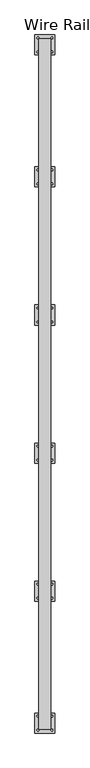
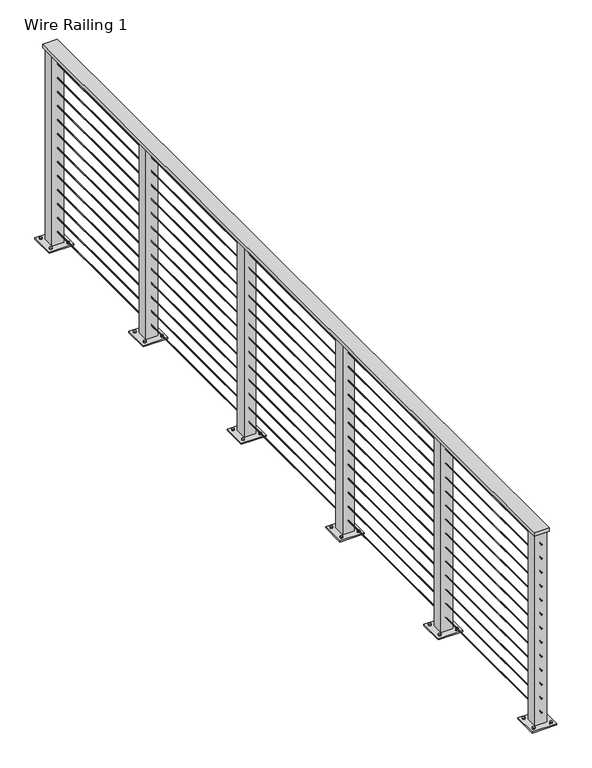
"""IFC4 building model written with IfcOpenShell, lengths in millimetres: railing geometry, Wire Railing 1."""

from ifc_helpers import new_model, si_unit, point, frame, frame_2d, origin, place, context, project, spatial, polyline, circle_curve, trimmed, segment, composite_curve, outline, extrude, source, transform, mapped, element, save


def wire_railing_1_9cbc15e5(model_context):
    return source(origin(), model_context, "Body", "SweptSolid", [
        extrude(outline(polyline([(33186.6840778, 35259.9668167), (33262.8840778, 35259.9668167), (33262.8840778, 30878.4668167), (33186.6840778, 30878.4668167), (33186.6840778, 35259.9668167)])), frame((0.0, 0.0, 270306.8), z_axis=(0.0, 0.0, 1.0), x_axis=(1.0, 0.0, 0.0)), (0.0, 0.0, 1.0), 19.05),
        extrude(outline(composite_curve([segment(trimmed(circle_curve(frame_2d((270247.26875, 33224.7840778)), 2.38125), [point((270247.26875, 33227.1653278))], [point((270247.26875, 33222.4028278))], False, "CARTESIAN"), True, "CONTINUOUS"), segment(trimmed(circle_curve(frame_2d((270247.26875, 33224.7840778)), 2.38125), [point((270247.26875, 33222.4028278))], [point((270247.26875, 33227.1653278))], False, "CARTESIAN"), True, "CONTINUOUS")], self_intersect=False)), frame((0.0, 30878.4668167, 0.0), z_axis=(0.0, 1.0, 0.0), x_axis=(0.0, 0.0, 1.0)), (0.0, 0.0, 1.0), 4381.5),
        extrude(outline(composite_curve([segment(trimmed(circle_curve(frame_2d((270171.06875, 33224.7840778)), 2.38125), [point((270171.06875, 33227.1653278))], [point((270171.06875, 33222.4028278))], False, "CARTESIAN"), True, "CONTINUOUS"), segment(trimmed(circle_curve(frame_2d((270171.06875, 33224.7840778)), 2.38125), [point((270171.06875, 33222.4028278))], [point((270171.06875, 33227.1653278))], False, "CARTESIAN"), True, "CONTINUOUS")], self_intersect=False)), frame((0.0, 30878.4668167, 0.0), z_axis=(0.0, 1.0, 0.0), x_axis=(0.0, 0.0, 1.0)), (0.0, 0.0, 1.0), 4381.5),
        extrude(outline(composite_curve([segment(trimmed(circle_curve(frame_2d((270094.86875, 33224.7840778)), 2.38125), [point((270094.86875, 33227.1653278))], [point((270094.86875, 33222.4028278))], False, "CARTESIAN"), True, "CONTINUOUS"), segment(trimmed(circle_curve(frame_2d((270094.86875, 33224.7840778)), 2.38125), [point((270094.86875, 33222.4028278))], [point((270094.86875, 33227.1653278))], False, "CARTESIAN"), True, "CONTINUOUS")], self_intersect=False)), frame((0.0, 30878.4668167, 0.0), z_axis=(0.0, 1.0, 0.0), x_axis=(0.0, 0.0, 1.0)), (0.0, 0.0, 1.0), 4381.5),
        extrude(outline(composite_curve([segment(trimmed(circle_curve(frame_2d((270018.66875, 33224.7840778)), 2.38125), [point((270018.66875, 33227.1653278))], [point((270018.66875, 33222.4028278))], False, "CARTESIAN"), True, "CONTINUOUS"), segment(trimmed(circle_curve(frame_2d((270018.66875, 33224.7840778)), 2.38125), [point((270018.66875, 33222.4028278))], [point((270018.66875, 33227.1653278))], False, "CARTESIAN"), True, "CONTINUOUS")], self_intersect=False)), frame((0.0, 30878.4668167, 0.0), z_axis=(0.0, 1.0, 0.0), x_axis=(0.0, 0.0, 1.0)), (0.0, 0.0, 1.0), 4381.5),
        extrude(outline(composite_curve([segment(trimmed(circle_curve(frame_2d((269942.46875, 33224.7840778)), 2.38125), [point((269942.46875, 33227.1653278))], [point((269942.46875, 33222.4028278))], False, "CARTESIAN"), True, "CONTINUOUS"), segment(trimmed(circle_curve(frame_2d((269942.46875, 33224.7840778)), 2.38125), [point((269942.46875, 33222.4028278))], [point((269942.46875, 33227.1653278))], False, "CARTESIAN"), True, "CONTINUOUS")], self_intersect=False)), frame((0.0, 30878.4668167, 0.0), z_axis=(0.0, 1.0, 0.0), x_axis=(0.0, 0.0, 1.0)), (0.0, 0.0, 1.0), 4381.5),
        extrude(outline(composite_curve([segment(trimmed(circle_curve(frame_2d((269866.26875, 33224.7840778)), 2.38125), [point((269866.26875, 33227.1653278))], [point((269866.26875, 33222.4028278))], False, "CARTESIAN"), True, "CONTINUOUS"), segment(trimmed(circle_curve(frame_2d((269866.26875, 33224.7840778)), 2.38125), [point((269866.26875, 33222.4028278))], [point((269866.26875, 33227.1653278))], False, "CARTESIAN"), True, "CONTINUOUS")], self_intersect=False)), frame((0.0, 30878.4668167, 0.0), z_axis=(0.0, 1.0, 0.0), x_axis=(0.0, 0.0, 1.0)), (0.0, 0.0, 1.0), 4381.5),
        extrude(outline(composite_curve([segment(trimmed(circle_curve(frame_2d((269790.06875, 33224.7840778)), 2.38125), [point((269790.06875, 33227.1653278))], [point((269790.06875, 33222.4028278))], False, "CARTESIAN"), True, "CONTINUOUS"), segment(trimmed(circle_curve(frame_2d((269790.06875, 33224.7840778)), 2.38125), [point((269790.06875, 33222.4028278))], [point((269790.06875, 33227.1653278))], False, "CARTESIAN"), True, "CONTINUOUS")], self_intersect=False)), frame((0.0, 30878.4668167, 0.0), z_axis=(0.0, 1.0, 0.0), x_axis=(0.0, 0.0, 1.0)), (0.0, 0.0, 1.0), 4381.5),
        extrude(outline(composite_curve([segment(trimmed(circle_curve(frame_2d((269713.86875, 33224.7840778)), 2.38125), [point((269713.86875, 33227.1653278))], [point((269713.86875, 33222.4028278))], False, "CARTESIAN"), True, "CONTINUOUS"), segment(trimmed(circle_curve(frame_2d((269713.86875, 33224.7840778)), 2.38125), [point((269713.86875, 33222.4028278))], [point((269713.86875, 33227.1653278))], False, "CARTESIAN"), True, "CONTINUOUS")], self_intersect=False)), frame((0.0, 30878.4668167, 0.0), z_axis=(0.0, 1.0, 0.0), x_axis=(0.0, 0.0, 1.0)), (0.0, 0.0, 1.0), 4381.5),
        extrude(outline(composite_curve([segment(trimmed(circle_curve(frame_2d((269637.66875, 33224.7840778)), 2.38125), [point((269637.66875, 33227.1653278))], [point((269637.66875, 33222.4028278))], False, "CARTESIAN"), True, "CONTINUOUS"), segment(trimmed(circle_curve(frame_2d((269637.66875, 33224.7840778)), 2.38125), [point((269637.66875, 33222.4028278))], [point((269637.66875, 33227.1653278))], False, "CARTESIAN"), True, "CONTINUOUS")], self_intersect=False)), frame((0.0, 30878.4668167, 0.0), z_axis=(0.0, 1.0, 0.0), x_axis=(0.0, 0.0, 1.0)), (0.0, 0.0, 1.0), 4381.5),
        extrude(outline(composite_curve([segment(trimmed(circle_curve(frame_2d((269561.46875, 33224.7840778)), 2.38125), [point((269561.46875, 33227.1653278))], [point((269561.46875, 33222.4028278))], False, "CARTESIAN"), True, "CONTINUOUS"), segment(trimmed(circle_curve(frame_2d((269561.46875, 33224.7840778)), 2.38125), [point((269561.46875, 33222.4028278))], [point((269561.46875, 33227.1653278))], False, "CARTESIAN"), True, "CONTINUOUS")], self_intersect=False)), frame((0.0, 30878.4668167, 0.0), z_axis=(0.0, 1.0, 0.0), x_axis=(0.0, 0.0, 1.0)), (0.0, 0.0, 1.0), 4381.5),
        extrude(outline(composite_curve([segment(trimmed(circle_curve(frame_2d((269485.26875, 33224.7840778)), 2.38125), [point((269485.26875, 33227.1653278))], [point((269485.26875, 33222.4028278))], False, "CARTESIAN"), True, "CONTINUOUS"), segment(trimmed(circle_curve(frame_2d((269485.26875, 33224.7840778)), 2.38125), [point((269485.26875, 33222.4028278))], [point((269485.26875, 33227.1653278))], False, "CARTESIAN"), True, "CONTINUOUS")], self_intersect=False)), frame((0.0, 30878.4668167, 0.0), z_axis=(0.0, 1.0, 0.0), x_axis=(0.0, 0.0, 1.0)), (0.0, 0.0, 1.0), 4381.5),
        extrude(outline(composite_curve([segment(trimmed(circle_curve(frame_2d((269409.06875, 33224.7840778)), 2.38125), [point((269409.06875, 33227.1653278))], [point((269409.06875, 33222.4028278))], False, "CARTESIAN"), True, "CONTINUOUS"), segment(trimmed(circle_curve(frame_2d((269409.06875, 33224.7840778)), 2.38125), [point((269409.06875, 33222.4028278))], [point((269409.06875, 33227.1653278))], False, "CARTESIAN"), True, "CONTINUOUS")], self_intersect=False)), frame((0.0, 30878.4668167, 0.0), z_axis=(0.0, 1.0, 0.0), x_axis=(0.0, 0.0, 1.0)), (0.0, 0.0, 1.0), 4381.5),
        extrude(outline(composite_curve([segment(trimmed(circle_curve(frame_2d((269332.86875, 33224.7840778)), 2.38125), [point((269332.86875, 33227.1653278))], [point((269332.86875, 33222.4028278))], False, "CARTESIAN"), True, "CONTINUOUS"), segment(trimmed(circle_curve(frame_2d((269332.86875, 33224.7840778)), 2.38125), [point((269332.86875, 33222.4028278))], [point((269332.86875, 33227.1653278))], False, "CARTESIAN"), True, "CONTINUOUS")], self_intersect=False)), frame((0.0, 30878.4668167, 0.0), z_axis=(0.0, 1.0, 0.0), x_axis=(0.0, 0.0, 1.0)), (0.0, 0.0, 1.0), 4381.5),
        extrude(outline(composite_curve([segment(trimmed(circle_curve(frame_2d((33180.3340778, 31799.2168167)), 6.35), [point((33173.9840778, 31799.2168167))], [point((33186.6840778, 31799.2168167))], False, "CARTESIAN"), True, "CONTINUOUS"), segment(trimmed(circle_curve(frame_2d((33180.3340778, 31799.2168167)), 6.35), [point((33186.6840778, 31799.2168167))], [point((33173.9840778, 31799.2168167))], False, "CARTESIAN"), True, "CONTINUOUS")], self_intersect=False)), frame((0.0, 0.0, 269259.05), z_axis=(0.0, 0.0, 1.0), x_axis=(1.0, 0.0, 0.0)), (0.0, 0.0, 1.0), 12.7),
        extrude(outline(composite_curve([segment(trimmed(circle_curve(frame_2d((33269.2340778, 31799.2168167)), 6.35), [point((33262.8840778, 31799.2168167))], [point((33275.5840778, 31799.2168167))], False, "CARTESIAN"), True, "CONTINUOUS"), segment(trimmed(circle_curve(frame_2d((33269.2340778, 31799.2168167)), 6.35), [point((33275.5840778, 31799.2168167))], [point((33262.8840778, 31799.2168167))], False, "CARTESIAN"), True, "CONTINUOUS")], self_intersect=False)), frame((0.0, 0.0, 269259.05), z_axis=(0.0, 0.0, 1.0), x_axis=(1.0, 0.0, 0.0)), (0.0, 0.0, 1.0), 12.7),
        extrude(outline(composite_curve([segment(trimmed(circle_curve(frame_2d((33180.3340778, 31710.3168167)), 6.35), [point((33173.9840778, 31710.3168167))], [point((33186.6840778, 31710.3168167))], False, "CARTESIAN"), True, "CONTINUOUS"), segment(trimmed(circle_curve(frame_2d((33180.3340778, 31710.3168167)), 6.35), [point((33186.6840778, 31710.3168167))], [point((33173.9840778, 31710.3168167))], False, "CARTESIAN"), True, "CONTINUOUS")], self_intersect=False)), frame((0.0, 0.0, 269259.05), z_axis=(0.0, 0.0, 1.0), x_axis=(1.0, 0.0, 0.0)), (0.0, 0.0, 1.0), 12.7),
        extrude(outline(composite_curve([segment(trimmed(circle_curve(frame_2d((33269.2340778, 31710.3168167)), 6.35), [point((33262.8840778, 31710.3168167))], [point((33275.5840778, 31710.3168167))], False, "CARTESIAN"), True, "CONTINUOUS"), segment(trimmed(circle_curve(frame_2d((33269.2340778, 31710.3168167)), 6.35), [point((33275.5840778, 31710.3168167))], [point((33262.8840778, 31710.3168167))], False, "CARTESIAN"), True, "CONTINUOUS")], self_intersect=False)), frame((0.0, 0.0, 269259.05), z_axis=(0.0, 0.0, 1.0), x_axis=(1.0, 0.0, 0.0)), (0.0, 0.0, 1.0), 12.7),
        extrude(outline(polyline([(33288.2840778, 31818.2668167), (33288.2840778, 31691.2668167), (33161.2840778, 31691.2668167), (33161.2840778, 31818.2668167), (33288.2840778, 31818.2668167)])), frame((0.0, 0.0, 269259.05), z_axis=(0.0, 0.0, 1.0), x_axis=(1.0, 0.0, 0.0)), (0.0, 0.0, 1.0), 6.35),
        extrude(outline(polyline([(33254.9465778, 31784.9293167), (33254.9465778, 31724.6043167), (33194.6215778, 31724.6043167), (33194.6215778, 31784.9293167), (33254.9465778, 31784.9293167)]), holes=[polyline([(33248.5965778, 31778.5793167), (33200.9715778, 31778.5793167), (33200.9715778, 31730.9543167), (33248.5965778, 31730.9543167), (33248.5965778, 31778.5793167)])]), frame((0.0, 0.0, 269259.05), z_axis=(0.0, 0.0, 1.0), x_axis=(1.0, 0.0, 0.0)), (0.0, 0.0, 1.0), 1047.75),
        extrude(outline(composite_curve([segment(trimmed(circle_curve(frame_2d((33180.3340778, 32675.5168167)), 6.35), [point((33173.9840778, 32675.5168167))], [point((33186.6840778, 32675.5168167))], False, "CARTESIAN"), True, "CONTINUOUS"), segment(trimmed(circle_curve(frame_2d((33180.3340778, 32675.5168167)), 6.35), [point((33186.6840778, 32675.5168167))], [point((33173.9840778, 32675.5168167))], False, "CARTESIAN"), True, "CONTINUOUS")], self_intersect=False)), frame((0.0, 0.0, 269259.05), z_axis=(0.0, 0.0, 1.0), x_axis=(1.0, 0.0, 0.0)), (0.0, 0.0, 1.0), 12.7),
        extrude(outline(composite_curve([segment(trimmed(circle_curve(frame_2d((33269.2340778, 32675.5168167)), 6.35), [point((33262.8840778, 32675.5168167))], [point((33275.5840778, 32675.5168167))], False, "CARTESIAN"), True, "CONTINUOUS"), segment(trimmed(circle_curve(frame_2d((33269.2340778, 32675.5168167)), 6.35), [point((33275.5840778, 32675.5168167))], [point((33262.8840778, 32675.5168167))], False, "CARTESIAN"), True, "CONTINUOUS")], self_intersect=False)), frame((0.0, 0.0, 269259.05), z_axis=(0.0, 0.0, 1.0), x_axis=(1.0, 0.0, 0.0)), (0.0, 0.0, 1.0), 12.7),
        extrude(outline(composite_curve([segment(trimmed(circle_curve(frame_2d((33180.3340778, 32586.6168167)), 6.35), [point((33173.9840778, 32586.6168167))], [point((33186.6840778, 32586.6168167))], False, "CARTESIAN"), True, "CONTINUOUS"), segment(trimmed(circle_curve(frame_2d((33180.3340778, 32586.6168167)), 6.35), [point((33186.6840778, 32586.6168167))], [point((33173.9840778, 32586.6168167))], False, "CARTESIAN"), True, "CONTINUOUS")], self_intersect=False)), frame((0.0, 0.0, 269259.05), z_axis=(0.0, 0.0, 1.0), x_axis=(1.0, 0.0, 0.0)), (0.0, 0.0, 1.0), 12.7),
        extrude(outline(composite_curve([segment(trimmed(circle_curve(frame_2d((33269.2340778, 32586.6168167)), 6.35), [point((33262.8840778, 32586.6168167))], [point((33275.5840778, 32586.6168167))], False, "CARTESIAN"), True, "CONTINUOUS"), segment(trimmed(circle_curve(frame_2d((33269.2340778, 32586.6168167)), 6.35), [point((33275.5840778, 32586.6168167))], [point((33262.8840778, 32586.6168167))], False, "CARTESIAN"), True, "CONTINUOUS")], self_intersect=False)), frame((0.0, 0.0, 269259.05), z_axis=(0.0, 0.0, 1.0), x_axis=(1.0, 0.0, 0.0)), (0.0, 0.0, 1.0), 12.7),
        extrude(outline(polyline([(33288.2840778, 32694.5668167), (33288.2840778, 32567.5668167), (33161.2840778, 32567.5668167), (33161.2840778, 32694.5668167), (33288.2840778, 32694.5668167)])), frame((0.0, 0.0, 269259.05), z_axis=(0.0, 0.0, 1.0), x_axis=(1.0, 0.0, 0.0)), (0.0, 0.0, 1.0), 6.35),
        extrude(outline(polyline([(33254.9465778, 32661.2293167), (33254.9465778, 32600.9043167), (33194.6215778, 32600.9043167), (33194.6215778, 32661.2293167), (33254.9465778, 32661.2293167)]), holes=[polyline([(33248.5965778, 32654.8793167), (33200.9715778, 32654.8793167), (33200.9715778, 32607.2543167), (33248.5965778, 32607.2543167), (33248.5965778, 32654.8793167)])]), frame((0.0, 0.0, 269259.05), z_axis=(0.0, 0.0, 1.0), x_axis=(1.0, 0.0, 0.0)), (0.0, 0.0, 1.0), 1047.75),
        extrude(outline(composite_curve([segment(trimmed(circle_curve(frame_2d((33180.3340778, 33551.8168167)), 6.35), [point((33173.9840778, 33551.8168167))], [point((33186.6840778, 33551.8168167))], False, "CARTESIAN"), True, "CONTINUOUS"), segment(trimmed(circle_curve(frame_2d((33180.3340778, 33551.8168167)), 6.35), [point((33186.6840778, 33551.8168167))], [point((33173.9840778, 33551.8168167))], False, "CARTESIAN"), True, "CONTINUOUS")], self_intersect=False)), frame((0.0, 0.0, 269259.05), z_axis=(0.0, 0.0, 1.0), x_axis=(1.0, 0.0, 0.0)), (0.0, 0.0, 1.0), 12.7),
        extrude(outline(composite_curve([segment(trimmed(circle_curve(frame_2d((33269.2340778, 33551.8168167)), 6.35), [point((33262.8840778, 33551.8168167))], [point((33275.5840778, 33551.8168167))], False, "CARTESIAN"), True, "CONTINUOUS"), segment(trimmed(circle_curve(frame_2d((33269.2340778, 33551.8168167)), 6.35), [point((33275.5840778, 33551.8168167))], [point((33262.8840778, 33551.8168167))], False, "CARTESIAN"), True, "CONTINUOUS")], self_intersect=False)), frame((0.0, 0.0, 269259.05), z_axis=(0.0, 0.0, 1.0), x_axis=(1.0, 0.0, 0.0)), (0.0, 0.0, 1.0), 12.7),
        extrude(outline(composite_curve([segment(trimmed(circle_curve(frame_2d((33180.3340778, 33462.9168167)), 6.35), [point((33173.9840778, 33462.9168167))], [point((33186.6840778, 33462.9168167))], False, "CARTESIAN"), True, "CONTINUOUS"), segment(trimmed(circle_curve(frame_2d((33180.3340778, 33462.9168167)), 6.35), [point((33186.6840778, 33462.9168167))], [point((33173.9840778, 33462.9168167))], False, "CARTESIAN"), True, "CONTINUOUS")], self_intersect=False)), frame((0.0, 0.0, 269259.05), z_axis=(0.0, 0.0, 1.0), x_axis=(1.0, 0.0, 0.0)), (0.0, 0.0, 1.0), 12.7),
        extrude(outline(composite_curve([segment(trimmed(circle_curve(frame_2d((33269.2340778, 33462.9168167)), 6.35), [point((33262.8840778, 33462.9168167))], [point((33275.5840778, 33462.9168167))], False, "CARTESIAN"), True, "CONTINUOUS"), segment(trimmed(circle_curve(frame_2d((33269.2340778, 33462.9168167)), 6.35), [point((33275.5840778, 33462.9168167))], [point((33262.8840778, 33462.9168167))], False, "CARTESIAN"), True, "CONTINUOUS")], self_intersect=False)), frame((0.0, 0.0, 269259.05), z_axis=(0.0, 0.0, 1.0), x_axis=(1.0, 0.0, 0.0)), (0.0, 0.0, 1.0), 12.7),
        extrude(outline(polyline([(33288.2840778, 33570.8668167), (33288.2840778, 33443.8668167), (33161.2840778, 33443.8668167), (33161.2840778, 33570.8668167), (33288.2840778, 33570.8668167)])), frame((0.0, 0.0, 269259.05), z_axis=(0.0, 0.0, 1.0), x_axis=(1.0, 0.0, 0.0)), (0.0, 0.0, 1.0), 6.35),
        extrude(outline(polyline([(33254.9465778, 33537.5293167), (33254.9465778, 33477.2043167), (33194.6215778, 33477.2043167), (33194.6215778, 33537.5293167), (33254.9465778, 33537.5293167)]), holes=[polyline([(33248.5965778, 33531.1793167), (33200.9715778, 33531.1793167), (33200.9715778, 33483.5543167), (33248.5965778, 33483.5543167), (33248.5965778, 33531.1793167)])]), frame((0.0, 0.0, 269259.05), z_axis=(0.0, 0.0, 1.0), x_axis=(1.0, 0.0, 0.0)), (0.0, 0.0, 1.0), 1047.75),
        extrude(outline(composite_curve([segment(trimmed(circle_curve(frame_2d((33180.3340778, 34428.1168167)), 6.35), [point((33173.9840778, 34428.1168167))], [point((33186.6840778, 34428.1168167))], False, "CARTESIAN"), True, "CONTINUOUS"), segment(trimmed(circle_curve(frame_2d((33180.3340778, 34428.1168167)), 6.35), [point((33186.6840778, 34428.1168167))], [point((33173.9840778, 34428.1168167))], False, "CARTESIAN"), True, "CONTINUOUS")], self_intersect=False)), frame((0.0, 0.0, 269259.05), z_axis=(0.0, 0.0, 1.0), x_axis=(1.0, 0.0, 0.0)), (0.0, 0.0, 1.0), 12.7),
        extrude(outline(composite_curve([segment(trimmed(circle_curve(frame_2d((33269.2340778, 34428.1168167)), 6.35), [point((33262.8840778, 34428.1168167))], [point((33275.5840778, 34428.1168167))], False, "CARTESIAN"), True, "CONTINUOUS"), segment(trimmed(circle_curve(frame_2d((33269.2340778, 34428.1168167)), 6.35), [point((33275.5840778, 34428.1168167))], [point((33262.8840778, 34428.1168167))], False, "CARTESIAN"), True, "CONTINUOUS")], self_intersect=False)), frame((0.0, 0.0, 269259.05), z_axis=(0.0, 0.0, 1.0), x_axis=(1.0, 0.0, 0.0)), (0.0, 0.0, 1.0), 12.7),
        extrude(outline(composite_curve([segment(trimmed(circle_curve(frame_2d((33180.3340778, 34339.2168167)), 6.35), [point((33173.9840778, 34339.2168167))], [point((33186.6840778, 34339.2168167))], False, "CARTESIAN"), True, "CONTINUOUS"), segment(trimmed(circle_curve(frame_2d((33180.3340778, 34339.2168167)), 6.35), [point((33186.6840778, 34339.2168167))], [point((33173.9840778, 34339.2168167))], False, "CARTESIAN"), True, "CONTINUOUS")], self_intersect=False)), frame((0.0, 0.0, 269259.05), z_axis=(0.0, 0.0, 1.0), x_axis=(1.0, 0.0, 0.0)), (0.0, 0.0, 1.0), 12.7),
        extrude(outline(composite_curve([segment(trimmed(circle_curve(frame_2d((33269.2340778, 34339.2168167)), 6.35), [point((33262.8840778, 34339.2168167))], [point((33275.5840778, 34339.2168167))], False, "CARTESIAN"), True, "CONTINUOUS"), segment(trimmed(circle_curve(frame_2d((33269.2340778, 34339.2168167)), 6.35), [point((33275.5840778, 34339.2168167))], [point((33262.8840778, 34339.2168167))], False, "CARTESIAN"), True, "CONTINUOUS")], self_intersect=False)), frame((0.0, 0.0, 269259.05), z_axis=(0.0, 0.0, 1.0), x_axis=(1.0, 0.0, 0.0)), (0.0, 0.0, 1.0), 12.7),
        extrude(outline(polyline([(33288.2840778, 34447.1668167), (33288.2840778, 34320.1668167), (33161.2840778, 34320.1668167), (33161.2840778, 34447.1668167), (33288.2840778, 34447.1668167)])), frame((0.0, 0.0, 269259.05), z_axis=(0.0, 0.0, 1.0), x_axis=(1.0, 0.0, 0.0)), (0.0, 0.0, 1.0), 6.35),
        extrude(outline(polyline([(33254.9465778, 34413.8293167), (33254.9465778, 34353.5043167), (33194.6215778, 34353.5043167), (33194.6215778, 34413.8293167), (33254.9465778, 34413.8293167)]), holes=[polyline([(33248.5965778, 34407.4793167), (33200.9715778, 34407.4793167), (33200.9715778, 34359.8543167), (33248.5965778, 34359.8543167), (33248.5965778, 34407.4793167)])]), frame((0.0, 0.0, 269259.05), z_axis=(0.0, 0.0, 1.0), x_axis=(1.0, 0.0, 0.0)), (0.0, 0.0, 1.0), 1047.75),
        extrude(outline(composite_curve([segment(trimmed(circle_curve(frame_2d((33180.3340778, 30961.0168167)), 6.35), [point((33173.9840778, 30961.0168167))], [point((33186.6840778, 30961.0168167))], False, "CARTESIAN"), True, "CONTINUOUS"), segment(trimmed(circle_curve(frame_2d((33180.3340778, 30961.0168167)), 6.35), [point((33186.6840778, 30961.0168167))], [point((33173.9840778, 30961.0168167))], False, "CARTESIAN"), True, "CONTINUOUS")], self_intersect=False)), frame((0.0, 0.0, 269259.05), z_axis=(0.0, 0.0, 1.0), x_axis=(1.0, 0.0, 0.0)), (0.0, 0.0, 1.0), 12.7),
        extrude(outline(composite_curve([segment(trimmed(circle_curve(frame_2d((33269.2340778, 30961.0168167)), 6.35), [point((33262.8840778, 30961.0168167))], [point((33275.5840778, 30961.0168167))], False, "CARTESIAN"), True, "CONTINUOUS"), segment(trimmed(circle_curve(frame_2d((33269.2340778, 30961.0168167)), 6.35), [point((33275.5840778, 30961.0168167))], [point((33262.8840778, 30961.0168167))], False, "CARTESIAN"), True, "CONTINUOUS")], self_intersect=False)), frame((0.0, 0.0, 269259.05), z_axis=(0.0, 0.0, 1.0), x_axis=(1.0, 0.0, 0.0)), (0.0, 0.0, 1.0), 12.7),
        extrude(outline(composite_curve([segment(trimmed(circle_curve(frame_2d((33180.3340778, 30872.1168167)), 6.35), [point((33173.9840778, 30872.1168167))], [point((33186.6840778, 30872.1168167))], False, "CARTESIAN"), True, "CONTINUOUS"), segment(trimmed(circle_curve(frame_2d((33180.3340778, 30872.1168167)), 6.35), [point((33186.6840778, 30872.1168167))], [point((33173.9840778, 30872.1168167))], False, "CARTESIAN"), True, "CONTINUOUS")], self_intersect=False)), frame((0.0, 0.0, 269259.05), z_axis=(0.0, 0.0, 1.0), x_axis=(1.0, 0.0, 0.0)), (0.0, 0.0, 1.0), 12.7),
        extrude(outline(composite_curve([segment(trimmed(circle_curve(frame_2d((33269.2340778, 30872.1168167)), 6.35), [point((33262.8840778, 30872.1168167))], [point((33275.5840778, 30872.1168167))], False, "CARTESIAN"), True, "CONTINUOUS"), segment(trimmed(circle_curve(frame_2d((33269.2340778, 30872.1168167)), 6.35), [point((33275.5840778, 30872.1168167))], [point((33262.8840778, 30872.1168167))], False, "CARTESIAN"), True, "CONTINUOUS")], self_intersect=False)), frame((0.0, 0.0, 269259.05), z_axis=(0.0, 0.0, 1.0), x_axis=(1.0, 0.0, 0.0)), (0.0, 0.0, 1.0), 12.7),
        extrude(outline(polyline([(33288.2840778, 30980.0668167), (33288.2840778, 30853.0668167), (33161.2840778, 30853.0668167), (33161.2840778, 30980.0668167), (33288.2840778, 30980.0668167)])), frame((0.0, 0.0, 269259.05), z_axis=(0.0, 0.0, 1.0), x_axis=(1.0, 0.0, 0.0)), (0.0, 0.0, 1.0), 6.35),
        extrude(outline(polyline([(33254.9465778, 30946.7293167), (33254.9465778, 30886.4043167), (33194.6215778, 30886.4043167), (33194.6215778, 30946.7293167), (33254.9465778, 30946.7293167)]), holes=[polyline([(33248.5965778, 30940.3793167), (33200.9715778, 30940.3793167), (33200.9715778, 30892.7543167), (33248.5965778, 30892.7543167), (33248.5965778, 30940.3793167)])]), frame((0.0, 0.0, 269259.05), z_axis=(0.0, 0.0, 1.0), x_axis=(1.0, 0.0, 0.0)), (0.0, 0.0, 1.0), 1047.75),
        extrude(outline(composite_curve([segment(trimmed(circle_curve(frame_2d((33180.3340778, 35266.3168167)), 6.35), [point((33173.9840778, 35266.3168167))], [point((33186.6840778, 35266.3168167))], False, "CARTESIAN"), True, "CONTINUOUS"), segment(trimmed(circle_curve(frame_2d((33180.3340778, 35266.3168167)), 6.35), [point((33186.6840778, 35266.3168167))], [point((33173.9840778, 35266.3168167))], False, "CARTESIAN"), True, "CONTINUOUS")], self_intersect=False)), frame((0.0, 0.0, 269259.05), z_axis=(0.0, 0.0, 1.0), x_axis=(1.0, 0.0, 0.0)), (0.0, 0.0, 1.0), 12.7),
        extrude(outline(composite_curve([segment(trimmed(circle_curve(frame_2d((33269.2340778, 35266.3168167)), 6.35), [point((33262.8840778, 35266.3168167))], [point((33275.5840778, 35266.3168167))], False, "CARTESIAN"), True, "CONTINUOUS"), segment(trimmed(circle_curve(frame_2d((33269.2340778, 35266.3168167)), 6.35), [point((33275.5840778, 35266.3168167))], [point((33262.8840778, 35266.3168167))], False, "CARTESIAN"), True, "CONTINUOUS")], self_intersect=False)), frame((0.0, 0.0, 269259.05), z_axis=(0.0, 0.0, 1.0), x_axis=(1.0, 0.0, 0.0)), (0.0, 0.0, 1.0), 12.7),
        extrude(outline(composite_curve([segment(trimmed(circle_curve(frame_2d((33180.3340778, 35177.4168167)), 6.35), [point((33173.9840778, 35177.4168167))], [point((33186.6840778, 35177.4168167))], False, "CARTESIAN"), True, "CONTINUOUS"), segment(trimmed(circle_curve(frame_2d((33180.3340778, 35177.4168167)), 6.35), [point((33186.6840778, 35177.4168167))], [point((33173.9840778, 35177.4168167))], False, "CARTESIAN"), True, "CONTINUOUS")], self_intersect=False)), frame((0.0, 0.0, 269259.05), z_axis=(0.0, 0.0, 1.0), x_axis=(1.0, 0.0, 0.0)), (0.0, 0.0, 1.0), 12.7),
        extrude(outline(composite_curve([segment(trimmed(circle_curve(frame_2d((33269.2340778, 35177.4168167)), 6.35), [point((33262.8840778, 35177.4168167))], [point((33275.5840778, 35177.4168167))], False, "CARTESIAN"), True, "CONTINUOUS"), segment(trimmed(circle_curve(frame_2d((33269.2340778, 35177.4168167)), 6.35), [point((33275.5840778, 35177.4168167))], [point((33262.8840778, 35177.4168167))], False, "CARTESIAN"), True, "CONTINUOUS")], self_intersect=False)), frame((0.0, 0.0, 269259.05), z_axis=(0.0, 0.0, 1.0), x_axis=(1.0, 0.0, 0.0)), (0.0, 0.0, 1.0), 12.7),
        extrude(outline(polyline([(33288.2840778, 35285.3668167), (33288.2840778, 35158.3668167), (33161.2840778, 35158.3668167), (33161.2840778, 35285.3668167), (33288.2840778, 35285.3668167)])), frame((0.0, 0.0, 269259.05), z_axis=(0.0, 0.0, 1.0), x_axis=(1.0, 0.0, 0.0)), (0.0, 0.0, 1.0), 6.35),
        extrude(outline(polyline([(33254.9465778, 35252.0293167), (33254.9465778, 35191.7043167), (33194.6215778, 35191.7043167), (33194.6215778, 35252.0293167), (33254.9465778, 35252.0293167)]), holes=[polyline([(33248.5965778, 35245.6793167), (33200.9715778, 35245.6793167), (33200.9715778, 35198.0543167), (33248.5965778, 35198.0543167), (33248.5965778, 35245.6793167)])]), frame((0.0, 0.0, 269259.05), z_axis=(0.0, 0.0, 1.0), x_axis=(1.0, 0.0, 0.0)), (0.0, 0.0, 1.0), 1047.75),
    ])


if __name__ == "__main__":
    model = new_model("IFC4")
    model_context = context("Model", 3, world=origin())
    ifc_project = project(units=[si_unit("LENGTHUNIT", "METRE", prefix="MILLI")], contexts=[model_context])
    site = spatial("IfcSite", under=ifc_project)
    building = spatial("IfcBuilding", under=site)
    placement = place(None, origin())
    wire_railing_1_shape = wire_railing_1_9cbc15e5(model_context)
    element("IfcRailing", 1, ObjectType="Wire Railing 1", at=placement, inside=building, context=model_context, shape_type="MappedRepresentation", body=[
        mapped(wire_railing_1_shape, transform((0.0, 0.0, 0.0), x_axis=(1.0, 0.0, 0.0), y_axis=(0.0, 1.0, 0.0), z_axis=(0.0, 0.0, 1.0))),
    ])
    save(model, "model.ifc")

# Revit data of these elements
# Element 1 (IfcRailing, "Wire Railing 1")
#   Materials on its faces: "2 1/2\" X 2 1/2\" ALUM. SQUARE POST (38\" O.C. MAX)", "WIRE RAILING (3\" O.C.)", "ALUM. PLATE TOP RAIL"
# Materials
#   "2 1/2\" X 2 1/2\" ALUM. SQUARE POST (38\" O.C. MAX)": class "Metal", colour RGB 244 244 244, transparency 0, Manufacturer = "Kawneer", URL = "http://www.kawneer.com/kawneer/north_america/en/home.asp", Cost = 0
#   "WIRE RAILING (3\" O.C.)": class "Metal", colour RGB 244 244 244, transparency 0, Manufacturer = "Kawneer", URL = "http://www.kawneer.com/kawneer/north_america/en/home.asp", Cost = 0
#   "ALUM. PLATE TOP RAIL": class "Metal", colour RGB 244 244 244, transparency 0, Manufacturer = "Kawneer", URL = "http://www.kawneer.com/kawneer/north_america/en/home.asp", Cost = 0
